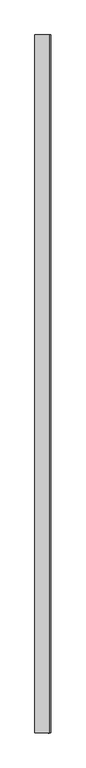
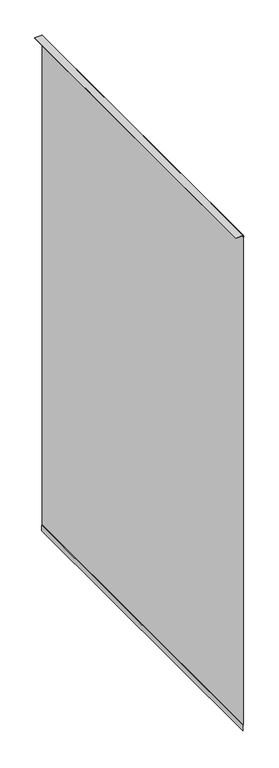
"""IFC4 building model written with IfcOpenShell, lengths in millimetres: proxy geometry, Generic Models 7:Generic Models 1:5:Generic Models 1:5 : Generic Models 7:Generic Models 1:337419:14 : Generic Models 7:Generic Models 1:5:Generic Models 1:5 : Generic Models 7:Generic Models 1:337419:311462."""

from ifc_helpers import new_model, si_unit, frame, origin, place, context, project, spatial, polyline, outline, extrude, source, transform, mapped, element, save


def generic_models_222c22bf(model_context):
    return source(origin(), model_context, "Body", "SweptSolid", [
        extrude(outline(polyline([(3723.8950904, 560351.4676125), (3721.7962359, 560301.0951049), (3720.2101121, 560301.1611934), (3722.2689531, 560350.5733762), (3714.8378379, 560354.8637326), (3705.2504916, 560351.3742239), (91.698248, 560351.3742239), (86.5070888, 560347.7393351), (46.3753703, 560347.7393351), (46.3753703, 560349.3268351), (86.006552, 560349.3268351), (91.1977111, 560352.9617239), (3704.9705725, 560352.9617239), (3714.990501, 560356.6086796), (3723.8950904, 560351.4676125)])), frame((0.0, -545634.6163841, 0.0), z_axis=(0.0, 1.0, 0.0), x_axis=(0.0, 0.0, 1.0)), (0.0, 0.0, 1.0), 2451.1),
    ])


if __name__ == "__main__":
    model = new_model("IFC4")
    model_context = context("Model", 3, world=origin())
    ifc_project = project(units=[si_unit("LENGTHUNIT", "METRE", prefix="MILLI")], contexts=[model_context])
    site = spatial("IfcSite", under=ifc_project)
    building = spatial("IfcBuilding", under=site)
    placement = place(None, origin())
    generic_models_shape = generic_models_222c22bf(model_context)
    element("IfcBuildingElementProxy", 1, Name="Generic Models 7:Generic Models 1:5:Generic Models 1:5 : Generic Models 7:Generic Models 1:337419:14 : Generic Models 7:Generic Models 1:5:Generic Models 1:5 : Generic Models 7:Generic Models 1:337419:311462", ObjectType="Generic Models 7:Generic Models 1:5:Generic Models 1:5 : Generic Models 7:Generic Models 1:337419:14 : Generic Models 7:Generic Models 1:5:Generic Models 1:5 : Generic Models 7:Generic Models 1:337419:311462", at=placement, inside=building, context=model_context, shape_type="MappedRepresentation", body=[
        mapped(generic_models_shape, transform((0.0, 0.0, 0.0), x_axis=(1.0, 0.0, 0.0), y_axis=(0.0, 1.0, 0.0), z_axis=(0.0, 0.0, 1.0))),
    ])
    save(model, "model.ifc")

# Revit data of these elements
# Type "Generic Models 7:Generic Models 1:5:Generic Models 1:5 : Generic Models 7:Generic Models 1:337419:14 : Generic Models 7:Generic Models 1:5:Generic Models 1:5 : Generic Models 7:Generic Models 1:337419:311462"
#   NameOverride = "Generic Models 7:Generic Models 1:5:Generic Models 1:5 : Generic Models 7:Generic Models 1:337419:311462"
#   ObjectTypeOverride = "Generic Models 1:5 : Generic Models 7:Generic Models 1:337419"
#   Reference = "Generic Models 1"
#   Tag = "311462"
# Element 1 (IfcBuildingElementProxy, "Generic Models 7:Generic Models 1:5:Generic Models 1:5 : Generic Models 7:Generic Models 1:337419:14 : Generic Models 7:Generic Models 1:5:Generic Models 1:5 : Generic Models 7:Generic Models 1:337419:311462")
#   Materials on its faces: "UV STABLE WATER RESISTANT VAPOR PERMEABLE AIR BARRIER (WRB) - WRAP JAMBS/HEADERS - BLACK COLOR"
# Materials
#   "UV STABLE WATER RESISTANT VAPOR PERMEABLE AIR BARRIER (WRB) - WRAP JAMBS/HEADERS - BLACK COLOR": class "Generic", colour RGB 51 162 45, transparency 0, Description = "Polyethylene film membrane", Cost = 0
